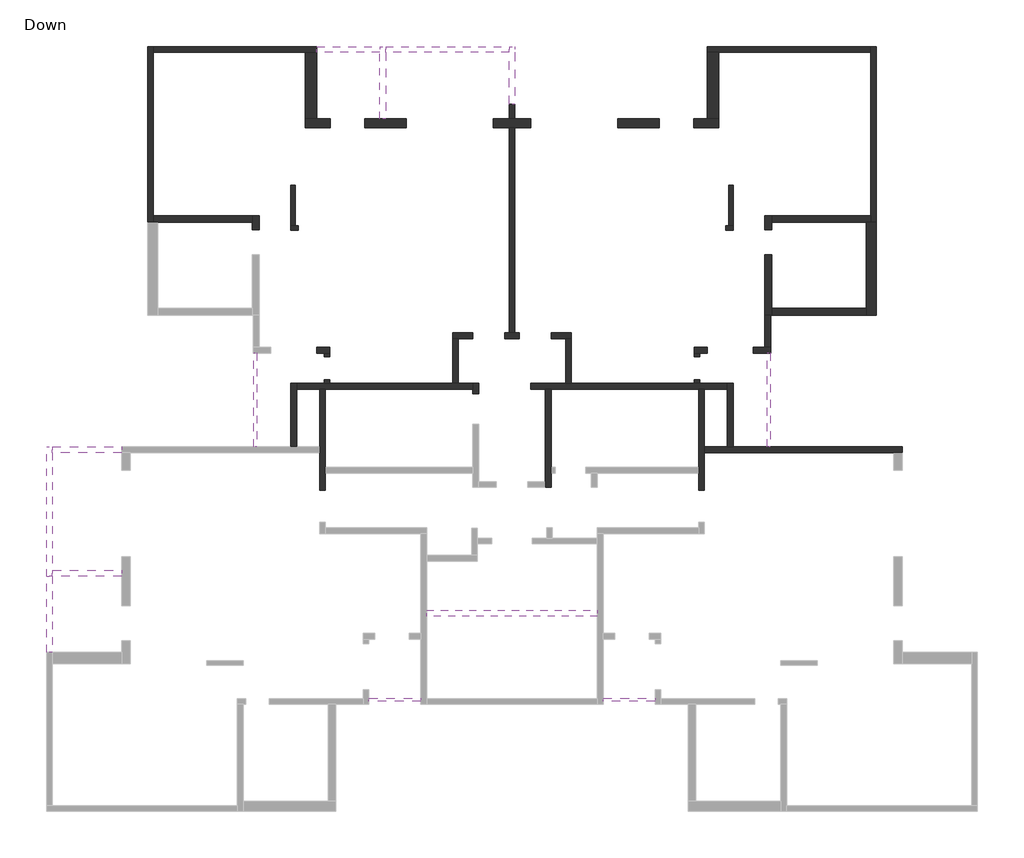
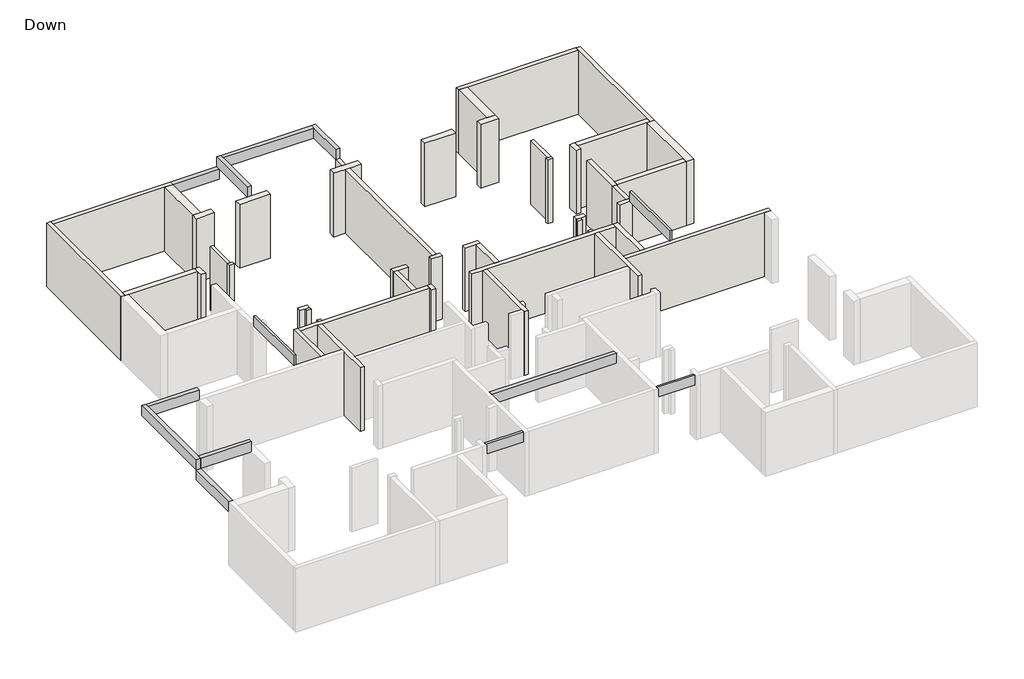
# One storey, part 2 of 2: 46 walls, 13 beams.
# Revit data of these elements (continued)
# Element 14 (IfcWall, "15") (continued)
#   Phase Created = New Construction
#   Base Constraint = Down
#   Top Constraint = Typical Floor
#   Materials on its faces: "Concrete"
# Element 15 (IfcWall, "15")
#   IfcGUID = "1e7LVzuKbECxrDX1g1kHc1"
#   Comments = ""
#   Mark = "W93"
#   SOFiSTiK_EdgeZones = "W84"
#   SOFiSTiK_AMG_Comments = ""
#   Top Offset = 0 cm
#   Base Offset = 0 cm
#   wall height = 318 cm
#   SOFiSTiK_AMG_Scheduled = yes
#   SOFiSTiK_AMG_Adjusted = yes
#   Phase Created = New Construction
#   Base Constraint = Down
#   Top Constraint = Typical Floor
#   Materials on its faces: "Concrete"
# Element 16 (IfcWall, "15")
#   IfcGUID = "3brXM_Qu1DvOaG$o2DBD0k"
#   Comments = ""
#   Mark = "W95"
#   SOFiSTiK_EdgeZones = "W86"
#   SOFiSTiK_AMG_Comments = ""
#   Top Offset = 0 cm
#   Base Offset = 0 cm
#   wall height = 318 cm
#   SOFiSTiK_AMG_Scheduled = yes
#   SOFiSTiK_AMG_Adjusted = yes
#   Phase Created = New Construction
#   Base Constraint = Down
#   Top Constraint = Typical Floor
#   Materials on its faces: "Concrete"
# Element 17 (IfcWall, "15")
#   IfcGUID = "3brXM_Qu1DvOaG$o2DBD0G"
#   Comments = ""
#   Mark = "W96"
#   SOFiSTiK_EdgeZones = "W87"
#   SOFiSTiK_AMG_Comments = ""
#   Top Offset = 0 cm
#   Base Offset = 0 cm
#   wall height = 318 cm
#   SOFiSTiK_AMG_Scheduled = yes
#   SOFiSTiK_AMG_Adjusted = yes
#   Phase Created = New Construction
#   Base Constraint = Down
#   Top Constraint = Typical Floor
#   Materials on its faces: "Concrete"
# Element 18 (IfcWall, "20")
#   IfcGUID = "1e7LVzuKbECxrDX1g1kMd3"
#   Comments = ""
#   Mark = "W1"
#   SOFiSTiK_EdgeZones = "W1"
#   SOFiSTiK_AMG_Comments = ""
#   Top Offset = 0 cm
#   Base Offset = 0 cm
#   wall height = 318 cm
#   SOFiSTiK_AMG_Scheduled = yes
#   SOFiSTiK_AMG_Adjusted = yes
#   Phase Created = New Construction
#   Base Constraint = Down
#   Top Constraint = Typical Floor
#   Materials on its faces: "Concrete"
# Element 19 (IfcWall, "20")
#   IfcGUID = "1e7LVzuKbECxrDX1g1kHEu"
#   Comments = ""
#   Mark = "W4"
#   SOFiSTiK_EdgeZones = "W4"
#   SOFiSTiK_AMG_Comments = ""
#   Top Offset = 0 cm
#   Base Offset = 0 cm
#   wall height = 318 cm
#   SOFiSTiK_AMG_Scheduled = yes
#   SOFiSTiK_AMG_Adjusted = yes
#   Phase Created = New Construction
#   Base Constraint = Down
#   Top Constraint = Typical Floor
#   Materials on its faces: "Concrete"
# Element 20 (IfcWall, "20")
#   IfcGUID = "1e7LVzuKbECxrDX1g1kHF$"
#   Comments = ""
#   Mark = "W5"
#   SOFiSTiK_EdgeZones = "W5"
#   SOFiSTiK_AMG_Comments = "Too Short /"
#   Top Offset = 0 cm
#   Base Offset = 0 cm
#   wall height = 318 cm
#   SOFiSTiK_AMG_Scheduled = yes
#   SOFiSTiK_AMG_Adjusted = yes
#   Phase Created = New Construction
#   Base Constraint = Down
#   Top Constraint = Typical Floor
#   Materials on its faces: "Concrete"
# Element 21 (IfcWall, "20")
#   IfcGUID = "1e7LVzuKbECxrDX1g1kHDc"
#   Comments = ""
#   Mark = "W6"
#   SOFiSTiK_EdgeZones = "W6"
#   SOFiSTiK_AMG_Comments = "Too Short /"
#   Top Offset = 0 cm
#   Base Offset = 0 cm
#   wall height = 318 cm
#   SOFiSTiK_AMG_Scheduled = yes
#   SOFiSTiK_AMG_Adjusted = yes
#   Phase Created = New Construction
#   Base Constraint = Down
#   Top Constraint = Typical Floor
#   Materials on its faces: "Concrete"
# Element 22 (IfcWall, "20")
#   IfcGUID = "1e7LVzuKbECxrDX1g1kH9T"
#   Comments = ""
#   Mark = "W7"
#   SOFiSTiK_EdgeZones = "W7"
#   SOFiSTiK_AMG_Comments = ""
#   Top Offset = 0 cm
#   Base Offset = 0 cm
#   wall height = 318 cm
#   SOFiSTiK_AMG_Scheduled = yes
#   SOFiSTiK_AMG_Adjusted = yes
#   Phase Created = New Construction
#   Base Constraint = Down
#   Top Constraint = Typical Floor
#   Materials on its faces: "Concrete"
# Element 23 (IfcWall, "20")
#   IfcGUID = "1e7LVzuKbECxrDX1g1kH4v"
#   Comments = ""
#   Mark = "W8"
#   SOFiSTiK_EdgeZones = "W8"
#   SOFiSTiK_AMG_Comments = ""
#   Top Offset = 0 cm
#   Base Offset = 0 cm
#   wall height = 318 cm
#   SOFiSTiK_AMG_Scheduled = yes
#   SOFiSTiK_AMG_Adjusted = yes
#   Phase Created = New Construction
#   Base Constraint = Down
#   Top Constraint = Typical Floor
#   Materials on its faces: "Concrete"
# Element 24 (IfcWall, "20")
#   IfcGUID = "1e7LVzuKbECxrDX1g1kHPs"
#   Comments = ""
#   Mark = "W13"
#   SOFiSTiK_EdgeZones = "W12"
#   SOFiSTiK_AMG_Comments = ""
#   Top Offset = 0 cm
#   Base Offset = 0 cm
#   wall height = 318 cm
#   SOFiSTiK_AMG_Scheduled = yes
#   SOFiSTiK_AMG_Adjusted = yes
#   Phase Created = New Construction
#   Base Constraint = Down
#   Top Constraint = Typical Floor
#   Materials on its faces: "Concrete"
# Element 25 (IfcWall, "20")
#   IfcGUID = "1e7LVzuKbECxrDX1g1kHJf"
#   Comments = ""
#   Mark = "W15"
#   SOFiSTiK_EdgeZones = "W13"
#   SOFiSTiK_AMG_Comments = ""
#   Top Offset = 0 cm
#   Base Offset = 0 cm
#   wall height = 318 cm
#   SOFiSTiK_AMG_Scheduled = yes
#   SOFiSTiK_AMG_Adjusted = yes
#   Phase Created = New Construction
#   Base Constraint = Down
#   Top Constraint = Typical Floor
#   Materials on its faces: "Concrete"
# Element 26 (IfcWall, "20")
#   IfcGUID = "1e7LVzuKbECxrDX1g1kHbk"
#   Comments = ""
#   Mark = "W18"
#   SOFiSTiK_EdgeZones = "W15"
#   SOFiSTiK_AMG_Comments = ""
#   Top Offset = 0 cm
#   Base Offset = 0 cm
#   wall height = 318 cm
#   SOFiSTiK_AMG_Scheduled = yes
#   SOFiSTiK_AMG_Adjusted = yes
#   Phase Created = New Construction
#   Base Constraint = Down
#   Top Constraint = Typical Floor
#   Materials on its faces: "Concrete"
# Element 27 (IfcWall, "20")
#   IfcGUID = "1e7LVzuKbECxrDX1g1kHtL"
#   Comments = ""
#   Mark = "W19"
#   SOFiSTiK_EdgeZones = "W16"
#   SOFiSTiK_AMG_Comments = ""
#   Top Offset = 0 cm
#   Base Offset = 0 cm
#   wall height = 318 cm
#   SOFiSTiK_AMG_Scheduled = yes
#   SOFiSTiK_AMG_Adjusted = yes
#   Phase Created = New Construction
#   Base Constraint = Down
#   Top Constraint = Typical Floor
#   Materials on its faces: "Concrete"
# Element 28 (IfcWall, "20")
#   IfcGUID = "1e7LVzuKbECxrDX1g1kHou"
#   Comments = ""
#   Mark = "W20"
#   SOFiSTiK_EdgeZones = "W17"
#   SOFiSTiK_AMG_Comments = ""
#   Top Offset = 0 cm
#   Base Offset = 0 cm
#   wall height = 318 cm
#   SOFiSTiK_AMG_Scheduled = yes
#   SOFiSTiK_AMG_Adjusted = yes
#   Phase Created = New Construction
#   Base Constraint = Down
#   Top Constraint = Typical Floor
#   Materials on its faces: "Concrete"
# Element 29 (IfcWall, "20")
#   IfcGUID = "1e7LVzuKbECxrDX1g1kGEy"
#   Comments = ""
#   Mark = "W21"
#   SOFiSTiK_EdgeZones = "W18"
#   SOFiSTiK_AMG_Comments = ""
#   Top Offset = 0 cm
#   Base Offset = 0 cm
#   wall height = 318 cm
#   SOFiSTiK_AMG_Scheduled = yes
#   SOFiSTiK_AMG_Adjusted = yes
#   Phase Created = New Construction
#   Base Constraint = Down
#   Top Constraint = Typical Floor
#   Materials on its faces: "Concrete"
# Element 30 (IfcWall, "20")
#   IfcGUID = "1e7LVzuKbECxrDX1g1kGCw"
#   Comments = ""
#   Mark = "W22"
#   SOFiSTiK_EdgeZones = "W19"
#   SOFiSTiK_AMG_Comments = ""
#   Top Offset = 0 cm
#   Base Offset = 0 cm
#   wall height = 318 cm
#   SOFiSTiK_AMG_Scheduled = yes
#   SOFiSTiK_AMG_Adjusted = yes
#   Phase Created = New Construction
#   Base Constraint = Down
#   Top Constraint = Typical Floor
#   Materials on its faces: "Concrete"
# Element 31 (IfcWall, "20")
#   IfcGUID = "1e7LVzuKbECxrDX1g1kGAN"
#   Comments = ""
#   Mark = "W23"
#   SOFiSTiK_EdgeZones = "W20"
#   SOFiSTiK_AMG_Comments = ""
#   Top Offset = 0 cm
#   Base Offset = 0 cm
#   wall height = 318 cm
#   SOFiSTiK_AMG_Scheduled = yes
#   SOFiSTiK_AMG_Adjusted = yes
#   Phase Created = New Construction
#   Base Constraint = Down
#   Top Constraint = Typical Floor
#   Materials on its faces: "Concrete"
# Element 32 (IfcWall, "20")
#   IfcGUID = "3brXM_Qu1DvOaG$o2DBDV2"
#   Comments = ""
#   Mark = "W37"
#   SOFiSTiK_EdgeZones = "W33"
#   SOFiSTiK_AMG_Comments = ""
#   Top Offset = 0 cm
#   Base Offset = 0 cm
#   wall height = 318 cm
#   SOFiSTiK_AMG_Scheduled = yes
#   SOFiSTiK_AMG_Adjusted = yes
#   Phase Created = New Construction
#   Base Constraint = Down
#   Top Constraint = Typical Floor
#   Materials on its faces: "Concrete"
# Element 33 (IfcWall, "20")
#   IfcGUID = "3brXM_Qu1DvOaG$o2DBDVE"
#   Comments = ""
#   Mark = "W38"
#   SOFiSTiK_EdgeZones = "W34"
#   SOFiSTiK_AMG_Comments = ""
#   Top Offset = 0 cm
#   Base Offset = 0 cm
#   wall height = 318 cm
#   SOFiSTiK_AMG_Scheduled = yes
#   SOFiSTiK_AMG_Adjusted = yes
#   Phase Created = New Construction
#   Base Constraint = Down
#   Top Constraint = Typical Floor
#   Materials on its faces: "Concrete"
# Element 34 (IfcWall, "20")
#   IfcGUID = "3brXM_Qu1DvOaG$o2DBD0m"
#   Comments = ""
#   Mark = "W39"
#   SOFiSTiK_EdgeZones = "W35"
#   SOFiSTiK_AMG_Comments = ""
#   Top Offset = 0 cm
#   Base Offset = 0 cm
#   wall height = 318 cm
#   SOFiSTiK_AMG_Scheduled = yes
#   SOFiSTiK_AMG_Adjusted = yes
#   Phase Created = New Construction
#   Base Constraint = Down
#   Top Constraint = Typical Floor
#   Materials on its faces: "Concrete"
# Element 35 (IfcWall, "20")
#   IfcGUID = "3brXM_Qu1DvOaG$o2DBD0o"
#   Comments = ""
#   Mark = "W40"
#   SOFiSTiK_EdgeZones = "W36"
#   SOFiSTiK_AMG_Comments = ""
#   Top Offset = 0 cm
#   Base Offset = 0 cm
#   wall height = 318 cm
#   SOFiSTiK_AMG_Scheduled = yes
#   SOFiSTiK_AMG_Adjusted = yes
#   Phase Created = New Construction
#   Base Constraint = Down
#   Top Constraint = Typical Floor
#   Materials on its faces: "Concrete"
# Element 36 (IfcWall, "20")
#   IfcGUID = "3brXM_Qu1DvOaG$o2DBD0q"
#   Comments = ""
#   Mark = "W41"
#   SOFiSTiK_EdgeZones = "W37"
#   SOFiSTiK_AMG_Comments = "Too Short /"
#   Top Offset = 0 cm
#   Base Offset = 0 cm
#   wall height = 318 cm
#   SOFiSTiK_AMG_Scheduled = yes
#   SOFiSTiK_AMG_Adjusted = yes
#   Phase Created = New Construction
#   Base Constraint = Down
#   Top Constraint = Typical Floor
#   Materials on its faces: "Concrete"
# Element 37 (IfcWall, "20")
#   IfcGUID = "3brXM_Qu1DvOaG$o2DBD0s"
#   Comments = ""
#   Mark = "W42"
#   SOFiSTiK_EdgeZones = "W38"
#   SOFiSTiK_AMG_Comments = "Too Short /"
#   Top Offset = 0 cm
#   Base Offset = 0 cm
#   wall height = 318 cm
#   SOFiSTiK_AMG_Scheduled = yes
#   SOFiSTiK_AMG_Adjusted = yes
#   Phase Created = New Construction
#   Base Constraint = Down
#   Top Constraint = Typical Floor
#   Materials on its faces: "Concrete"
# Element 38 (IfcWall, "20")
#   IfcGUID = "3brXM_Qu1DvOaG$o2DBD0u"
#   Comments = ""
#   Mark = "W43"
#   SOFiSTiK_EdgeZones = "W39"
#   SOFiSTiK_AMG_Comments = ""
#   Top Offset = 0 cm
#   Base Offset = 0 cm
#   wall height = 318 cm
#   SOFiSTiK_AMG_Scheduled = yes
#   SOFiSTiK_AMG_Adjusted = yes
#   Phase Created = New Construction
#   Base Constraint = Down
#   Top Constraint = Typical Floor
#   Materials on its faces: "Concrete"
# Element 39 (IfcWall, "20")
#   IfcGUID = "3brXM_Qu1DvOaG$o2DBD0w"
#   Comments = ""
#   Mark = "W44"
#   SOFiSTiK_EdgeZones = "W40"
#   SOFiSTiK_AMG_Comments = ""
#   Top Offset = 0 cm
#   Base Offset = 0 cm
#   wall height = 318 cm
#   SOFiSTiK_AMG_Scheduled = yes
#   SOFiSTiK_AMG_Adjusted = yes
#   Phase Created = New Construction
#   Base Constraint = Down
#   Top Constraint = Typical Floor
#   Materials on its faces: "Concrete"
# Element 40 (IfcWall, "20")
#   IfcGUID = "3brXM_Qu1DvOaG$o2DBD0a"
#   Comments = ""
#   Mark = "W49"
#   SOFiSTiK_EdgeZones = "W43"
#   SOFiSTiK_AMG_Comments = ""
#   Top Offset = 0 cm
#   Base Offset = 0 cm
#   wall height = 318 cm
#   SOFiSTiK_AMG_Scheduled = yes
#   SOFiSTiK_AMG_Adjusted = yes
#   Phase Created = New Construction
#   Base Constraint = Down
#   Top Constraint = Typical Floor
#   Materials on its faces: "Concrete"
# Element 41 (IfcWall, "20")
#   IfcGUID = "3brXM_Qu1DvOaG$o2DBD0e"
#   Comments = ""
#   Mark = "W51"
#   SOFiSTiK_EdgeZones = "W44"
#   SOFiSTiK_AMG_Comments = ""
#   Top Offset = 0 cm
#   Base Offset = 0 cm
#   wall height = 318 cm
#   SOFiSTiK_AMG_Scheduled = yes
#   SOFiSTiK_AMG_Adjusted = yes
#   Phase Created = New Construction
#   Base Constraint = Down
#   Top Constraint = Typical Floor
#   Materials on its faces: "Concrete"
# Element 42 (IfcWall, "20")
#   IfcGUID = "3brXM_Qu1DvOaG$o2DBD0i"
#   Comments = ""
#   Mark = "W53"
#   SOFiSTiK_EdgeZones = "W45"
#   SOFiSTiK_AMG_Comments = ""
#   Top Offset = 0 cm
#   Base Offset = 0 cm
#   wall height = 318 cm
#   SOFiSTiK_AMG_Scheduled = yes
#   SOFiSTiK_AMG_Adjusted = yes
#   Phase Created = New Construction
#   Base Constraint = Down
#   Top Constraint = Typical Floor
#   Materials on its faces: "Concrete"
# Element 43 (IfcWall, "20")
#   IfcGUID = "3brXM_Qu1DvOaG$o2DBD0I"
#   Comments = ""
#   Mark = "W54"
#   SOFiSTiK_EdgeZones = "W46"
#   SOFiSTiK_AMG_Comments = ""
#   Top Offset = 0 cm
#   Base Offset = 0 cm
#   wall height = 318 cm
#   SOFiSTiK_AMG_Scheduled = yes
#   SOFiSTiK_AMG_Adjusted = yes
#   Phase Created = New Construction
#   Base Constraint = Down
#   Top Constraint = Typical Floor
#   Materials on its faces: "Concrete"
# Element 44 (IfcWall, "20")
#   IfcGUID = "3brXM_Qu1DvOaG$o2DBD0Q"
#   Comments = ""
#   Mark = "W55"
#   SOFiSTiK_EdgeZones = "W47"
#   SOFiSTiK_AMG_Comments = ""
#   Top Offset = 0 cm
#   Base Offset = 0 cm
#   wall height = 318 cm
#   SOFiSTiK_AMG_Scheduled = yes
#   SOFiSTiK_AMG_Adjusted = yes
#   Phase Created = New Construction
#   Base Constraint = Down
#   Top Constraint = Typical Floor
#   Materials on its faces: "Concrete"
# Element 45 (IfcWall, "20")
#   IfcGUID = "3brXM_Qu1DvOaG$o2DBD0S"
#   Comments = ""
#   Mark = "W56"
#   SOFiSTiK_EdgeZones = "W48"
#   SOFiSTiK_AMG_Comments = ""
#   Top Offset = 0 cm
#   Base Offset = 0 cm
#   wall height = 318 cm
#   SOFiSTiK_AMG_Scheduled = yes
#   SOFiSTiK_AMG_Adjusted = yes
#   Phase Created = New Construction
#   Base Constraint = Down
#   Top Constraint = Typical Floor
#   Materials on its faces: "Concrete"
# Element 46 (IfcWall, "23")
#   IfcGUID = "1e7LVzuKbECxrDX1g1kMWL"
#   Comments = ""
#   Mark = "W78"
#   SOFiSTiK_EdgeZones = "W69"
#   SOFiSTiK_AMG_Comments = ""
#   Top Offset = 0 cm
#   Base Offset = 0 cm
#   wall height = 318 cm
#   SOFiSTiK_AMG_Scheduled = yes
#   SOFiSTiK_AMG_Adjusted = yes
#   Phase Created = New Construction
#   Base Constraint = Down
#   Top Constraint = Typical Floor
#   Materials on its faces: "Concrete"
# Element 47 (IfcWall, "23")
#   IfcGUID = "1e7LVzuKbECxrDX1g1kMXR"
#   Comments = ""
#   Mark = "W79"
#   SOFiSTiK_EdgeZones = "W70"
#   SOFiSTiK_AMG_Comments = ""
#   Top Offset = 0 cm
#   Base Offset = 0 cm
#   wall height = 318 cm
#   SOFiSTiK_AMG_Scheduled = yes
#   SOFiSTiK_AMG_Adjusted = yes
#   Phase Created = New Construction
#   Base Constraint = Down
#   Top Constraint = Typical Floor
#   Materials on its faces: "Concrete"
# Element 48 (IfcWall, "23")
#   IfcGUID = "3brXM_Qu1DvOaG$o2DBDV4"
#   Comments = ""
#   Mark = "W81"
#   SOFiSTiK_EdgeZones = "W72"
#   SOFiSTiK_AMG_Comments = ""
#   Top Offset = 0 cm
#   Base Offset = 0 cm
#   wall height = 318 cm
#   SOFiSTiK_AMG_Scheduled = yes
#   SOFiSTiK_AMG_Adjusted = yes
#   Phase Created = New Construction
#   Base Constraint = Down
#   Top Constraint = Typical Floor
#   Materials on its faces: "Concrete"
# Element 49 (IfcWall, "23")
#   IfcGUID = "3brXM_Qu1DvOaG$o2DBDV6"
#   Comments = ""
#   Mark = "W82"
#   SOFiSTiK_EdgeZones = "W73"
#   SOFiSTiK_AMG_Comments = ""
#   Top Offset = 0 cm
#   Base Offset = 0 cm
#   wall height = 318 cm
#   SOFiSTiK_AMG_Scheduled = yes
#   SOFiSTiK_AMG_Adjusted = yes
#   Phase Created = New Construction
#   Base Constraint = Down
#   Top Constraint = Typical Floor
#   Materials on its faces: "Concrete"
# Element 50 (IfcWall, "23")
#   IfcGUID = "3brXM_Qu1DvOaG$o2DBDV8"
#   Comments = ""
#   Mark = "W83"
#   SOFiSTiK_EdgeZones = "W74"
#   SOFiSTiK_AMG_Comments = ""
#   Top Offset = 0 cm
#   Base Offset = 0 cm
#   wall height = 318 cm
#   SOFiSTiK_AMG_Scheduled = yes
#   SOFiSTiK_AMG_Adjusted = yes
#   Phase Created = New Construction
#   Base Constraint = Down
#   Top Constraint = Typical Floor
#   Materials on its faces: "Concrete"
# Element 51 (IfcWall, "25")
#   IfcGUID = "3brXM_Qu1DvOaG$o2DBDVC"
#   Comments = ""
#   Mark = "W90"
#   SOFiSTiK_EdgeZones = "W81"
#   SOFiSTiK_AMG_Comments = ""
#   Top Offset = 0 cm
#   Base Offset = 0 cm
#   wall height = 318 cm
#   SOFiSTiK_AMG_Scheduled = yes
#   SOFiSTiK_AMG_Adjusted = yes
#   Phase Created = New Construction
#   Base Constraint = Down
#   Top Constraint = Typical Floor
#   Materials on its faces: "Concrete"
# Element 52 (IfcWall, "30")
#   IfcGUID = "1e7LVzuKbECxrDX1g1kHyV"
#   Comments = ""
#   Mark = "W102"
#   SOFiSTiK_EdgeZones = "W93"
#   SOFiSTiK_AMG_Comments = ""
#   Top Offset = 0 cm
#   Base Offset = 0 cm
#   wall height = 318 cm
#   SOFiSTiK_AMG_Scheduled = yes
#   SOFiSTiK_AMG_Adjusted = yes
#   Phase Created = New Construction
#   Base Constraint = Down
#   Top Constraint = Typical Floor
#   Materials on its faces: "Concrete"
# Element 53 (IfcWall, "30")
#   IfcGUID = "1e7LVzuKbECxrDX1g1kHxn"
#   Comments = ""
#   Mark = "W103"
#   SOFiSTiK_EdgeZones = "W94"
#   SOFiSTiK_AMG_Comments = ""
#   Top Offset = 0 cm
#   Base Offset = 0 cm
#   wall height = 318 cm
#   SOFiSTiK_AMG_Scheduled = yes
#   SOFiSTiK_AMG_Adjusted = yes
#   Phase Created = New Construction
#   Base Constraint = Down
#   Top Constraint = Typical Floor
#   Materials on its faces: "Concrete"
# Element 54 (IfcWall, "30")
#   IfcGUID = "1e7LVzuKbECxrDX1g1kHvY"
#   Comments = ""
#   Mark = "W104"
#   SOFiSTiK_EdgeZones = "W95"
#   SOFiSTiK_AMG_Comments = ""
#   Top Offset = 0 cm
#   Base Offset = 0 cm
#   wall height = 318 cm
#   SOFiSTiK_AMG_Scheduled = yes
#   SOFiSTiK_AMG_Adjusted = yes
#   Phase Created = New Construction
#   Base Constraint = Down
#   Top Constraint = Typical Floor
#   Materials on its faces: "Concrete"
# Element 55 (IfcWall, "30")
#   IfcGUID = "3brXM_Qu1DvOaG$o2DBD0M"
#   Comments = ""
#   Mark = "W108"
#   SOFiSTiK_EdgeZones = "W99"
#   SOFiSTiK_AMG_Comments = ""
#   Top Offset = 0 cm
#   Base Offset = 0 cm
#   wall height = 318 cm
#   SOFiSTiK_AMG_Scheduled = yes
#   SOFiSTiK_AMG_Adjusted = yes
#   Phase Created = New Construction
#   Base Constraint = Down
#   Top Constraint = Typical Floor
#   Materials on its faces: "Concrete"
# Element 56 (IfcWall, "30")
#   IfcGUID = "3brXM_Qu1DvOaG$o2DBD0O"
#   Comments = ""
#   Mark = "W109"
#   SOFiSTiK_EdgeZones = "W100"
#   SOFiSTiK_AMG_Comments = ""
#   Top Offset = 0 cm
#   Base Offset = 0 cm
#   wall height = 318 cm
#   SOFiSTiK_AMG_Scheduled = yes
#   SOFiSTiK_AMG_Adjusted = yes
#   Phase Created = New Construction
#   Base Constraint = Down
#   Top Constraint = Typical Floor
#   Materials on its faces: "Concrete"
# Element 57 (IfcWall, "35")
#   IfcGUID = "3brXM_Qu1DvOaG$o2DBDVA"
#   Comments = ""
#   Mark = "W86"
#   SOFiSTiK_EdgeZones = "W77"
#   SOFiSTiK_AMG_Comments = ""
#   Top Offset = 0 cm
#   Base Offset = 0 cm
#   wall height = 318 cm
#   SOFiSTiK_AMG_Scheduled = yes
#   SOFiSTiK_AMG_Adjusted = yes
#   Phase Created = New Construction
#   Base Constraint = Down
#   Top Constraint = Typical Floor
#   Materials on its faces: "Concrete"
# Element 58 (IfcWall, "40")
#   IfcGUID = "1e7LVzuKbECxrDX1g1kHXs"
#   Comments = ""
#   Mark = "W98"
#   SOFiSTiK_EdgeZones = "W89"
#   SOFiSTiK_AMG_Comments = ""
#   Top Offset = 0 cm
#   Base Offset = 0 cm
#   wall height = 318 cm
#   SOFiSTiK_AMG_Scheduled = yes
#   SOFiSTiK_AMG_Adjusted = yes
#   Phase Created = New Construction
#   Base Constraint = Down
#   Top Constraint = Typical Floor
#   Materials on its faces: "Concrete"
# Element 59 (IfcWall, "40")
#   IfcGUID = "3brXM_Qu1DvOaG$o2DBD0K"
#   Comments = ""
#   Mark = "W100"
#   SOFiSTiK_EdgeZones = "W91"
#   SOFiSTiK_AMG_Comments = ""
#   Top Offset = 0 cm
#   Base Offset = 0 cm
#   wall height = 318 cm
#   SOFiSTiK_AMG_Scheduled = yes
#   SOFiSTiK_AMG_Adjusted = yes
#   Phase Created = New Construction
#   Base Constraint = Down
#   Top Constraint = Typical Floor
#   Materials on its faces: "Concrete"
# Materials
#   "Concrete": class "Concrete", colour RGB 192 192 192, transparency 0, Keynote = "01000", Description = "Cast-in-place concrete", Cost = 0
